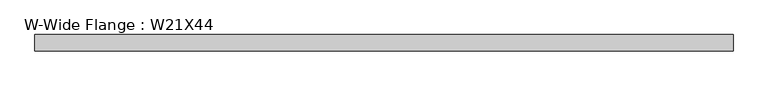
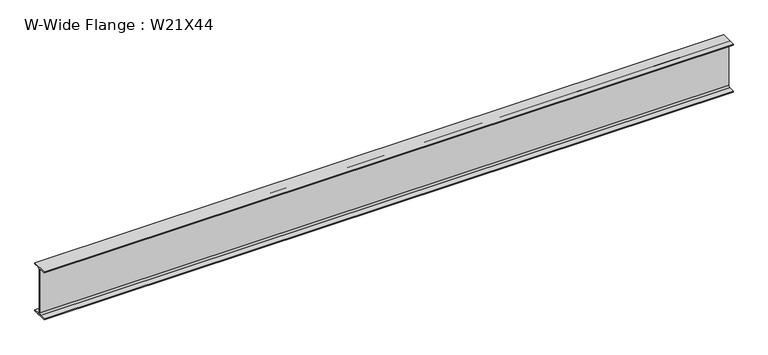
"""IFC4 building model written with IfcOpenShell, lengths in millimetres: beam geometry, W-Wide Flange : W21X44."""

from ifc_helpers import new_model, si_unit, point, frame, frame_2d, origin, place, context, project, spatial, polyline, circle_curve, trimmed, segment, composite_curve, outline, extrude, source, transform, mapped, element, save


def w_wide_flange_w21x44_84bfd685(model_context):
    return source(origin(), model_context, "Body", "SweptSolid", [
        extrude(outline(composite_curve([segment(polyline([(82.55, -251.46), (82.55, -262.89), (-82.55, -262.89), (-82.55, -251.46), (-21.59, -251.46)]), True, "CONTINUOUS"), segment(trimmed(circle_curve(frame_2d((-21.59, -234.315)), 17.145), [point((-21.59, -251.46))], [point((-4.445, -234.315))], True, "CARTESIAN"), True, "CONTINUOUS"), segment(polyline([(-4.445, -234.315), (-4.445, 234.315)]), True, "CONTINUOUS"), segment(trimmed(circle_curve(frame_2d((-21.59, 234.315)), 17.145), [point((-4.445, 234.315))], [point((-21.59, 251.46))], True, "CARTESIAN"), True, "CONTINUOUS"), segment(polyline([(-21.59, 251.46), (-82.55, 251.46), (-82.55, 262.89), (82.55, 262.89), (82.55, 251.46), (21.59, 251.46)]), True, "CONTINUOUS"), segment(trimmed(circle_curve(frame_2d((21.59, 234.315)), 17.145), [point((21.59, 251.46))], [point((4.445, 234.315))], True, "CARTESIAN"), True, "CONTINUOUS"), segment(polyline([(4.445, 234.315), (4.445, -234.315)]), True, "CONTINUOUS"), segment(trimmed(circle_curve(frame_2d((21.59, -234.315)), 17.145), [point((4.445, -234.315))], [point((21.59, -251.46))], True, "CARTESIAN"), True, "CONTINUOUS"), segment(polyline([(21.59, -251.46), (82.55, -251.46)]), True, "CONTINUOUS")], self_intersect=False)), frame((-3511.5003906, 0.0, 0.0), z_axis=(1.0, 0.0, 0.0), x_axis=(0.0, 1.0, 0.0)), (0.0, 0.0, 1.0), 7123.9836406),
    ])


if __name__ == "__main__":
    model = new_model("IFC4")
    model_context = context("Model", 3, world=origin())
    ifc_project = project(units=[si_unit("LENGTHUNIT", "METRE", prefix="MILLI")], contexts=[model_context])
    site = spatial("IfcSite", under=ifc_project)
    building = spatial("IfcBuilding", under=site)
    placement = place(None, origin())
    w_wide_flange_w21x44_shape = w_wide_flange_w21x44_84bfd685(model_context)
    element("IfcBeam", 1, ObjectType="W-Wide Flange : W21X44", at=placement, inside=building, context=model_context, shape_type="MappedRepresentation", body=[
        mapped(w_wide_flange_w21x44_shape, transform((0.0, 0.0, 0.0), x_axis=(1.0, 0.0, 0.0), y_axis=(0.0, 1.0, 0.0), z_axis=(0.0, 0.0, 1.0))),
    ])
    save(model, "model.ifc")

# Revit data of these elements
# Type "W-Wide Flange : W21X44"
#   Assembly Code = "B10"
#   W = 44
#   Length [instance default] = 1524 mm
#   bf = 165.1 mm
#   d = 525.78 mm
#   k = 28.575 mm
#   k2 = 17.145 mm
#   tf = 11.43 mm
#   tw = 8.89 mm
#   A = 0.00838708 m²
#   Structural Material [instance default] = Steel ASTM A992
# Element 1 (IfcBeam, "W-Wide Flange : W21X44")
#   Structural Material = Aluminum, Anodized Red
#   Materials on its faces: "Aluminum, Anodized Red"
# Materials
#   "Steel ASTM A992": class "Metal", colour RGB 128 0 0, transparency 0, Description = "Structural steel 50ksi", Cost = 0
#   "Aluminum, Anodized Red": class "Metal", colour RGB 120 120 120, transparency 0, Description = "Anodized aluminum, red", Cost = 0
